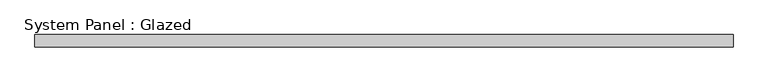
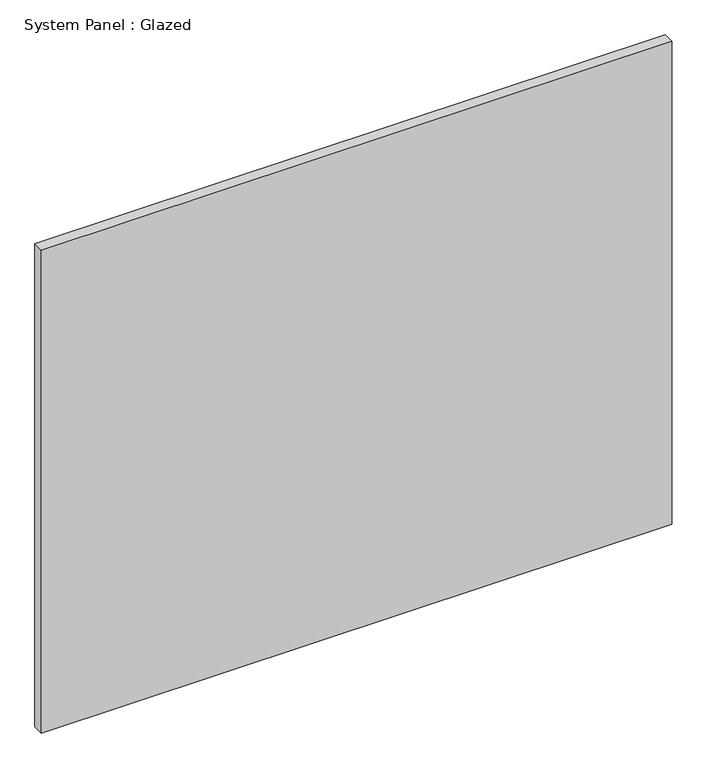
"""IFC4 building model written with IfcOpenShell, lengths in millimetres: plate geometry, System Panel : Glazed."""

from ifc_helpers import new_model, si_unit, origin, origin_with_axes, place, context, project, spatial, polyline, outline, extrude, source, transform, mapped, element, save


def system_panel_glazed_0adb819a(model_context):
    return source(origin(), model_context, "Body", "SweptSolid", [
        extrude(outline(polyline([(713.3166666, -44.45), (-713.3166666, -44.45), (-713.3166666, -19.05), (713.3166666, -19.05), (713.3166666, -44.45)])), origin_with_axes(), (0.0, 0.0, 1.0), 1155.7),
    ])


if __name__ == "__main__":
    model = new_model("IFC4")
    model_context = context("Model", 3, world=origin())
    ifc_project = project(units=[si_unit("LENGTHUNIT", "METRE", prefix="MILLI")], contexts=[model_context])
    site = spatial("IfcSite", under=ifc_project)
    building = spatial("IfcBuilding", under=site)
    placement = place(None, origin())
    system_panel_glazed_shape = system_panel_glazed_0adb819a(model_context)
    element("IfcPlate", 1, ObjectType="System Panel : Glazed", at=placement, inside=building, context=model_context, shape_type="MappedRepresentation", body=[
        mapped(system_panel_glazed_shape, transform((0.0, 0.0, 0.0), x_axis=(1.0, 0.0, 0.0), y_axis=(0.0, 1.0, 0.0), z_axis=(0.0, 0.0, 1.0))),
    ])
    save(model, "model.ifc")

# Revit data of these elements
# Type "System Panel : Glazed"
#   Construction Type Id = "GSP4R"
#   Analytic Construction = "1/8 in Pilkington single glazing"
#   Visual Light Transmittance = 0.9
#   Solar Heat Gain Coefficient = 0.86
#   Heat Transfer Coefficient (U) = 1.18115 BTU/(h·ft²·°F)
#   Define Thermal Properties by = 1
# Element 1 (IfcPlate, "System Panel : Glazed")
#   Materials on its faces: "Glass"
# Materials
#   "Glass": class "Glass", colour RGB 0 128 192, transparency 0.75, Description = "Soda Lime Glass", Cost = 0
